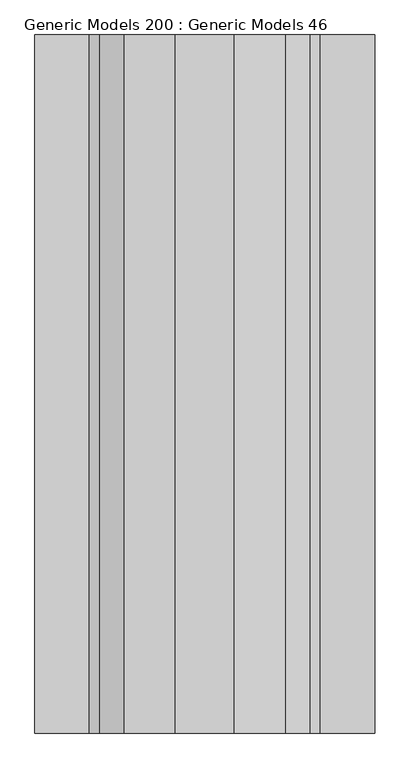
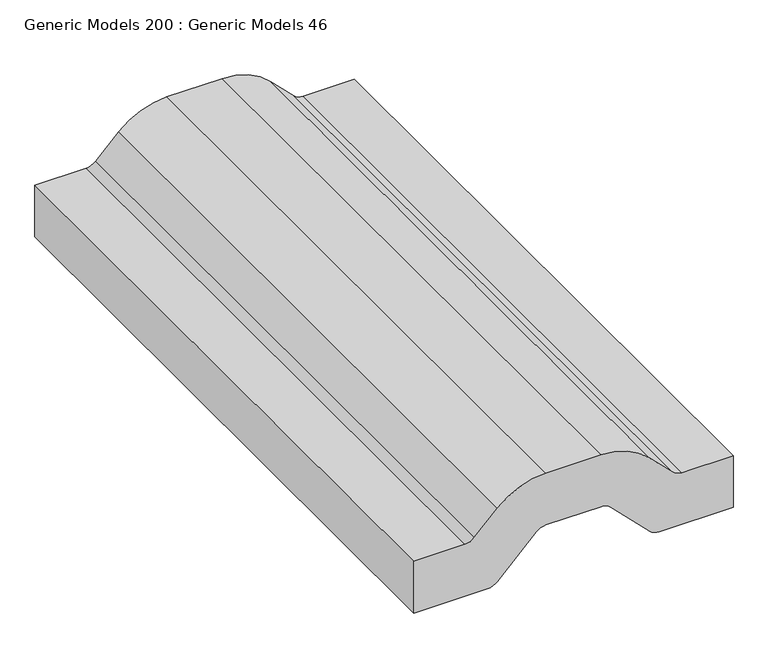
"""IFC4 building model written with IfcOpenShell, lengths in millimetres: proxy geometry, Generic Models 200 : Generic Models 46."""

from ifc_helpers import new_model, si_unit, point, frame, frame_2d, origin, place, context, project, spatial, polyline, circle_curve, trimmed, segment, composite_curve, outline, extrude, source, transform, mapped, element, save


def generic_models_200_generic_models_46_d53a038a(model_context):
    return source(origin(), model_context, "Body", "SweptSolid", [
        extrude(outline(composite_curve([segment(trimmed(circle_curve(frame_2d((2162.8204978, 47350.9539755)), 25.4), [point((2188.2204978, 47350.9539755))], [point((2180.7810101, 47368.9144878))], True, "CARTESIAN"), True, "CONTINUOUS"), segment(polyline([(2180.7810101, 47368.9144878), (2108.3699157, 47441.3255821)]), True, "CONTINUOUS"), segment(trimmed(circle_curve(frame_2d((2126.330428, 47459.2860944)), 25.4), [point((2108.3699157, 47441.3255821))], [point((2100.930428, 47459.2860944))], False, "CARTESIAN"), True, "CONTINUOUS"), segment(polyline([(2100.930428, 47459.2860944), (2100.930428, 47596.425), (2202.530428, 47596.425), (2202.530428, 47501.3701923)]), True, "CONTINUOUS"), segment(trimmed(circle_curve(frame_2d((2227.930428, 47501.3701923)), 25.4), [point((2202.530428, 47501.3701923))], [point((2209.9699157, 47483.4096801))], True, "CARTESIAN"), True, "CONTINUOUS"), segment(polyline([(2209.9699157, 47483.4096801), (2252.623059, 47440.7565367)]), True, "CONTINUOUS"), segment(trimmed(circle_curve(frame_2d((2162.8204978, 47350.9539755)), 127.0), [point((2252.623059, 47440.7565367))], [point((2289.8204978, 47350.9539755))], False, "CARTESIAN"), True, "CONTINUOUS"), segment(polyline([(2289.8204978, 47350.9539755), (2289.8204978, 47248.1710245)]), True, "CONTINUOUS"), segment(trimmed(circle_curve(frame_2d((2162.8204978, 47248.1710245)), 127.0), [point((2289.8204978, 47248.1710245))], [point((2252.623059, 47158.3684633))], False, "CARTESIAN"), True, "CONTINUOUS"), segment(polyline([(2252.623059, 47158.3684633), (2209.9699157, 47115.7153199)]), True, "CONTINUOUS"), segment(trimmed(circle_curve(frame_2d((2227.930428, 47097.7548077)), 25.4), [point((2209.9699157, 47115.7153199))], [point((2202.530428, 47097.7548077))], True, "CARTESIAN"), True, "CONTINUOUS"), segment(polyline([(2202.530428, 47097.7548077), (2202.530428, 47002.7), (2100.930428, 47002.7), (2100.930428, 47139.8389056)]), True, "CONTINUOUS"), segment(trimmed(circle_curve(frame_2d((2126.330428, 47139.8389056)), 25.4), [point((2100.930428, 47139.8389056))], [point((2108.3699157, 47157.7994179))], False, "CARTESIAN"), True, "CONTINUOUS"), segment(polyline([(2108.3699157, 47157.7994179), (2180.7810101, 47230.2105122)]), True, "CONTINUOUS"), segment(trimmed(circle_curve(frame_2d((2162.8204978, 47248.1710245)), 25.4), [point((2180.7810101, 47230.2105122))], [point((2188.2204978, 47248.1710245))], True, "CARTESIAN"), True, "CONTINUOUS"), segment(polyline([(2188.2204978, 47248.1710245), (2188.2204978, 47350.9539755)]), True, "CONTINUOUS")], self_intersect=False)), frame((0.0, 0.0, 0.0), z_axis=(0.0, 1.0, 0.0), x_axis=(0.0, 0.0, 1.0)), (0.0, 0.0, 1.0), 1219.2),
    ])


if __name__ == "__main__":
    model = new_model("IFC4")
    model_context = context("Model", 3, world=origin())
    ifc_project = project(units=[si_unit("LENGTHUNIT", "METRE", prefix="MILLI")], contexts=[model_context])
    site = spatial("IfcSite", under=ifc_project)
    building = spatial("IfcBuilding", under=site)
    placement = place(None, origin())
    generic_models_200_generic_models_46_shape = generic_models_200_generic_models_46_d53a038a(model_context)
    element("IfcBuildingElementProxy", 1, Name="Generic Models 200 : Generic Models 46", ObjectType="Generic Models 200 : Generic Models 46", at=placement, inside=building, context=model_context, shape_type="MappedRepresentation", body=[
        mapped(generic_models_200_generic_models_46_shape, transform((0.0, 0.0, 0.0), x_axis=(1.0, 0.0, 0.0), y_axis=(0.0, 1.0, 0.0), z_axis=(0.0, 0.0, 1.0))),
    ])
    save(model, "model.ifc")

# Revit data of these elements
# Element 1 (IfcBuildingElementProxy, "Generic Models 200 : Generic Models 46")
#   Materials on its faces: "BATT. INSULATION - EXTEND 4'-0\" MIN. - EACH SIDE OF STUD"
# Materials
#   "BATT. INSULATION - EXTEND 4'-0\" MIN. - EACH SIDE OF STUD": class "Unassigned", colour RGB 255 255 255, transparency 0, Cost = 0
